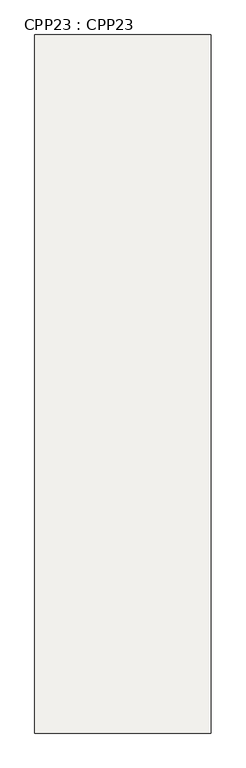
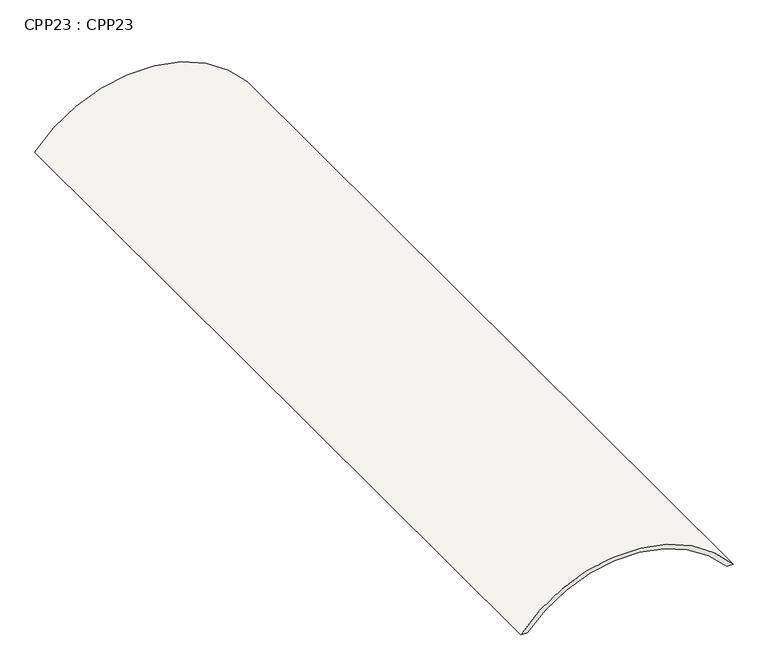
"""IFC4 building model written with IfcOpenShell, lengths in millimetres: slab geometry, CPP23 : CPP23."""

from ifc_helpers import new_model, si_unit, point, frame, frame_2d, origin, place, context, project, spatial, polyline, circle_curve, trimmed, segment, composite_curve, outline, extrude, source, transform, mapped, element, save


def cpp23_cpp23_ce2f35c4(model_context):
    return source(origin(), model_context, "Body", "SweptSolid", [
        extrude(outline(composite_curve([segment(polyline([(14620.0, 35333.2245514), (14620.0, 35483.2245514)]), True, "CONTINUOUS"), segment(trimmed(circle_curve(frame_2d((12603.2870371, 37833.2245514)), 3096.7129629), [point((14620.0, 35483.2245514))], [point((14620.0, 40183.2245513))], True, "CARTESIAN"), True, "CONTINUOUS"), segment(polyline([(14620.0, 40183.2245513), (14620.0, 40333.2245513)]), True, "CONTINUOUS"), segment(trimmed(circle_curve(frame_2d((12561.6949153, 37833.2245514)), 3238.3050847), [point((14620.0, 40333.2245513))], [point((14620.0, 35333.2245514))], False, "CARTESIAN"), True, "CONTINUOUS")], self_intersect=False)), frame((0.0, -100.2551788, 0.0), z_axis=(0.0, 1.0, 0.0), x_axis=(0.0, 0.0, 1.0)), (0.0, 0.0, 1.0), 19800.2551781),
    ])


if __name__ == "__main__":
    model = new_model("IFC4")
    model_context = context("Model", 3, world=origin())
    ifc_project = project(units=[si_unit("LENGTHUNIT", "METRE", prefix="MILLI")], contexts=[model_context])
    site = spatial("IfcSite", under=ifc_project)
    building = spatial("IfcBuilding", under=site)
    placement = place(None, origin())
    cpp23_cpp23_shape = cpp23_cpp23_ce2f35c4(model_context)
    element("IfcSlab", 1, ObjectType="CPP23 : CPP23", at=placement, inside=building, context=model_context, shape_type="MappedRepresentation", body=[
        mapped(cpp23_cpp23_shape, transform((0.0, 0.0, 0.0), x_axis=(1.0, 0.0, 0.0), y_axis=(0.0, 1.0, 0.0), z_axis=(0.0, 0.0, 1.0))),
    ])
    save(model, "model.ifc")

# Revit data of these elements
# Element 1 (IfcSlab, "CPP23 : CPP23")
#   Materials on its faces: "Concrete, RC"
# Materials
#   "Concrete, RC": class "Concrete", colour RGB 128 128 128, transparency 0, Description = "Cast-in-place concrete", Cost = 0
